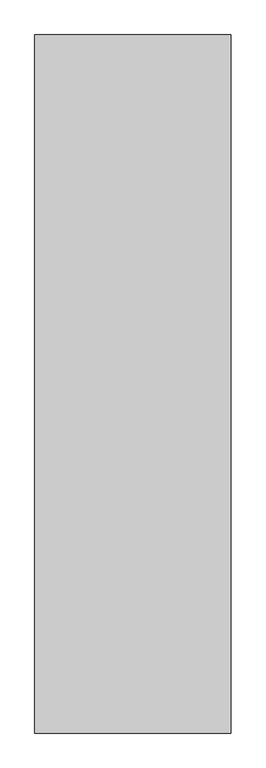
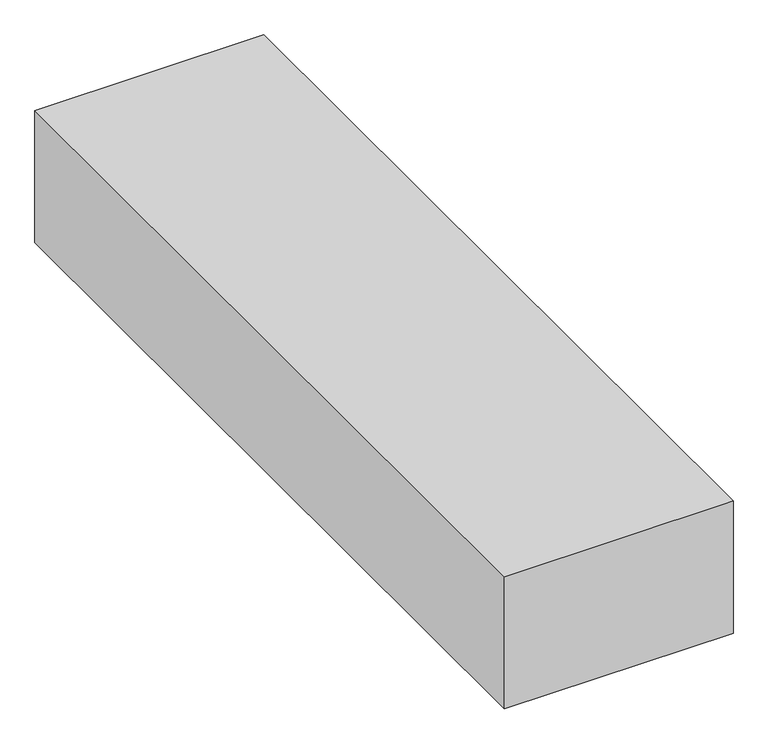
"""IFC4 building model written with IfcOpenShell, lengths in millimetres: proxy geometry, Space Planning Box_hec : Space Planning Box_hec."""

from ifc_helpers import new_model, si_unit, origin, origin_with_axes, place, context, project, spatial, polyline, outline, extrude, source, transform, mapped, element, save


def generic_models_50f5a469(model_context):
    return source(origin(), model_context, "Body", "SweptSolid", [
        extrude(outline(polyline([(4500.0, 16000.0), (4500.0, -16000.0), (-4500.0, -16000.0), (-4500.0, 16000.0), (4500.0, 16000.0)])), origin_with_axes(), (0.0, 0.0, 1.0), 5500.0),
    ])


if __name__ == "__main__":
    model = new_model("IFC4")
    model_context = context("Model", 3, world=origin())
    ifc_project = project(units=[si_unit("LENGTHUNIT", "METRE", prefix="MILLI")], contexts=[model_context])
    site = spatial("IfcSite", under=ifc_project)
    building = spatial("IfcBuilding", under=site)
    placement = place(None, origin())
    generic_models_shape = generic_models_50f5a469(model_context)
    element("IfcBuildingElementProxy", 1, Name="Space Planning Box_hec : Space Planning Box_hec", ObjectType="Space Planning Box_hec : Space Planning Box_hec", at=placement, inside=building, context=model_context, shape_type="MappedRepresentation", body=[
        mapped(generic_models_shape, transform((0.0, 0.0, 0.0), x_axis=(1.0, 0.0, 0.0), y_axis=(0.0, 1.0, 0.0), z_axis=(0.0, 0.0, 1.0))),
    ])
    save(model, "model.ifc")

# Revit data of these elements
# Type "Space Planning Box_hec : Space Planning Box_hec"
#   Type Comments = "..."
#   Room Name [instance default] = "?"
#   Interior Finish [instance default] = ""
#   Exterior Finish [instance default] = ""
#   Department [instance default] = ""
#   Assembly Code = "..."
#   ceiling height [instance default] = 0
#   Width [instance default] = 1524 mm
#   Program Area [instance default] = 0.00 m²
#   Length [instance default] = 1524 mm
#   Height [instance default] = 1524 mm
#   Area [instance default] = 2.32258 m²
#   Fill Color [instance default] = Cyan
#   Default Elevation = 0
# Element 1 (IfcBuildingElementProxy, "Space Planning Box_hec : Space Planning Box_hec")
#   Room Name = "Electrical Room-1"
#   Exterior Finish = "N/A..N/A,,EW1..EW2..N/A"
#   Department = "CI"
#   Width = 9000 mm
#   Program Area = 306.00 m²
#   Length = 32000 mm
#   Height = 5500 mm
#   Area = 288.00 m²
#   Fill Color = Yellow
#   Materials on its faces: "Yellow"
# Materials
#   "Cyan": class "Generic", colour RGB 0 255 255, transparency 0.2, Cost = 0
#   "Yellow": class "Generic", colour RGB 255 255 0, transparency 0.2, Cost = 0
